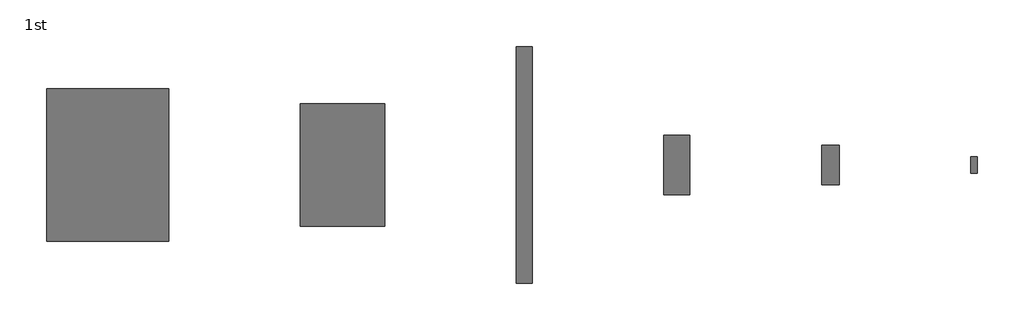
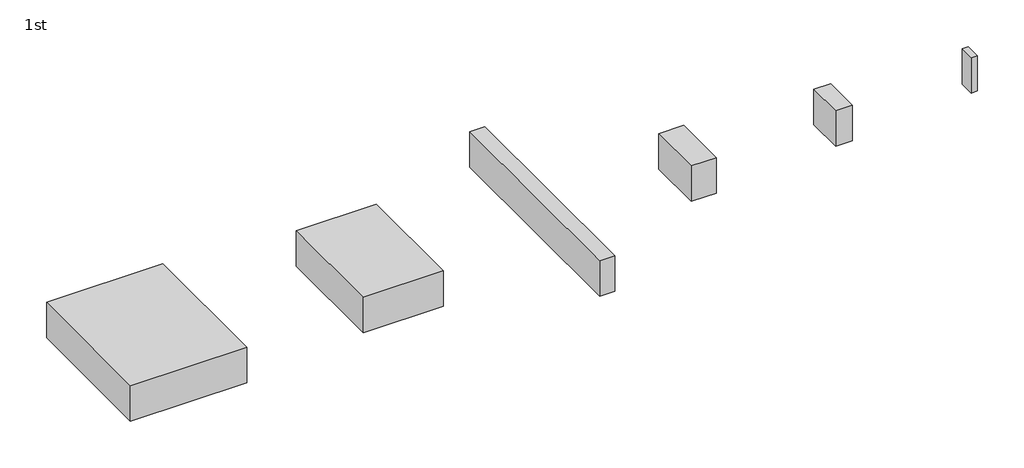
# One storey: 6 proxies.
"""IFC4 building model written with IfcOpenShell, lengths in millimetres."""

import ifcopenshell
import ifcopenshell.guid

model = None  # the IFC model being written
_history = None  # IfcOwnerHistory: only IFC2X3 demands one
_inside = {}  # id of a spatial element -> (the spatial element, [elements in it])
_under = {}  # id of a project, library or spatial element -> (it, [spatial elements below it])
_declared = {}  # id of a project -> (the project, [libraries it declares])
_typed = {}  # id of a type object -> (the type object, [elements of that type])
_made_of = {}  # id of a material, layer set ... -> (it, [elements and type objects made of it])


def new_model(schema):
    """Start an empty IFC model of exactly this schema.

    Asked for "IFC4X3", IfcOpenShell would pick the latest addendum, in which some entities
    have other attributes; the version numbers below select the first issue.
    IFC2X3 requires an IfcOwnerHistory on every rooted entity: one is made here for all.
    """
    global model, _history
    if schema == "IFC4X3":
        model = ifcopenshell.file(schema_version=(4, 3, 0, 0))
    else:
        model = ifcopenshell.file(schema=schema)
    _inside.clear()
    _under.clear()
    _declared.clear()
    _typed.clear()
    _made_of.clear()
    _history = None
    if model.schema == "IFC2X3":
        org = make("IfcOrganization", Name="unknown")
        user = make(
            "IfcPersonAndOrganization",
            ThePerson=make("IfcPerson", FamilyName="unknown"),
            TheOrganization=org,
        )
        app = make(
            "IfcApplication",
            ApplicationDeveloper=org,
            Version="unknown",
            ApplicationFullName="unknown",
            ApplicationIdentifier="unknown",
        )
        _history = make(
            "IfcOwnerHistory",
            OwningUser=user,
            OwningApplication=app,
            ChangeAction="ADDED",
            CreationDate=0,
        )
    return model


def make(cls, **values):
    """One entity of the class cls with the attributes given. An attribute that is None is left unset."""
    return model.create_entity(
        cls, **{name: value for name, value in values.items() if value is not None}
    )


def rooted(cls, **values):
    """An entity with a GlobalId (a new one), such as an element, a storey or a relation."""
    return make(cls, GlobalId=ifcopenshell.guid.new(), OwnerHistory=_history, **values)


def si_unit(unit_type, name, prefix=None):
    """IfcSIUnit, for example si_unit("LENGTHUNIT", "METRE", prefix="MILLI")."""
    return make("IfcSIUnit", UnitType=unit_type, Prefix=prefix, Name=name)


def assignment(units):
    """IfcUnitAssignment: the units of a project."""
    return None if units is None else make("IfcUnitAssignment", Units=units)


def point(xyz):
    """IfcCartesianPoint."""
    return None if xyz is None else make("IfcCartesianPoint", Coordinates=xyz)


def direction(xyz):
    """IfcDirection."""
    return None if xyz is None else make("IfcDirection", DirectionRatios=xyz)


def frame(location, z_axis=None, x_axis=None):
    """IfcAxis2Placement3D, a coordinate frame: its origin and axes. An axis left out is left unset."""
    return make(
        "IfcAxis2Placement3D",
        Location=point(location),
        Axis=direction(z_axis),
        RefDirection=direction(x_axis),
    )


def origin():
    """The frame at (0, 0, 0) with its axes left unset."""
    return frame((0.0, 0.0, 0.0))


def origin_with_axes():
    """The frame at (0, 0, 0) with the z axis (0, 0, 1) and the x axis (1, 0, 0) written out."""
    return frame((0.0, 0.0, 0.0), z_axis=(0.0, 0.0, 1.0), x_axis=(1.0, 0.0, 0.0))


def place(relative_to, where):
    """IfcLocalPlacement: puts the frame where relative to a parent placement (None: the world)."""
    return make(
        "IfcLocalPlacement", PlacementRelTo=relative_to, RelativePlacement=where
    )


def context(
    kind, dimensions, precision=None, world=None, true_north=None, identifier=None
):
    """IfcGeometricRepresentationContext, for example the 3D "Model" context."""
    return make(
        "IfcGeometricRepresentationContext",
        ContextIdentifier=identifier,
        ContextType=kind,
        CoordinateSpaceDimension=dimensions,
        Precision=precision,
        WorldCoordinateSystem=world,
        TrueNorth=true_north,
    )


def project(units=None, contexts=None):
    """IfcProject with its units and contexts."""
    return rooted(
        "IfcProject",
        Name="project",
        RepresentationContexts=contexts,
        UnitsInContext=assignment(units),
    )


def spatial(cls, under=None, at=None, **own):
    """A site, building, storey or space (cls), placed at a placement, below another one or the project."""
    s = rooted(cls, ObjectPlacement=at, **own)
    if under is not None:
        _under.setdefault(under.id(), (under, []))[1].append(s)
    return s


def polyline(points):
    """IfcPolyline through the points."""
    return make("IfcPolyline", Points=[point(p) for p in points])


def outline(outer, holes=None, kind="AREA"):
    """IfcArbitraryClosedProfileDef: a profile drawn as a closed curve; with holes, ...WithVoids."""
    if holes is None:
        return make("IfcArbitraryClosedProfileDef", ProfileType=kind, OuterCurve=outer)
    return make(
        "IfcArbitraryProfileDefWithVoids",
        ProfileType=kind,
        OuterCurve=outer,
        InnerCurves=holes,
    )


def extrude(swept, where, along, depth):
    """IfcExtrudedAreaSolid: the profile swept, set in the frame where, extruded along a direction by depth."""
    return make(
        "IfcExtrudedAreaSolid",
        SweptArea=swept,
        Position=where,
        ExtrudedDirection=direction(along),
        Depth=depth,
    )


def shape(context_of_items, identifier, shape_type, items):
    """IfcShapeRepresentation: the items that make up one representation, for example the "Body"."""
    return make(
        "IfcShapeRepresentation",
        ContextOfItems=context_of_items,
        RepresentationIdentifier=identifier,
        RepresentationType=shape_type,
        Items=items,
    )


def source(mapping_origin, context_of_items, identifier, shape_type, items):
    """IfcRepresentationMap: a shape defined once, which mapped items show again and again."""
    return make(
        "IfcRepresentationMap",
        MappingOrigin=mapping_origin,
        MappedRepresentation=shape(context_of_items, identifier, shape_type, items),
    )


def transform(
    local_origin,
    x_axis=None,
    y_axis=None,
    z_axis=None,
    scale=None,
    scale2=None,
    scale3=None,
    uniform=True,
):
    """IfcCartesianTransformationOperator3D, or its non-uniform kind. x_axis, y_axis, z_axis: its Axis1, 2, 3."""
    if uniform:
        return make(
            "IfcCartesianTransformationOperator3D",
            Axis1=direction(x_axis),
            Axis2=direction(y_axis),
            LocalOrigin=point(local_origin),
            Scale=scale,
            Axis3=direction(z_axis),
        )
    return make(
        "IfcCartesianTransformationOperator3DnonUniform",
        Axis1=direction(x_axis),
        Axis2=direction(y_axis),
        LocalOrigin=point(local_origin),
        Scale=scale,
        Axis3=direction(z_axis),
        Scale2=scale2,
        Scale3=scale3,
    )


def mapped(mapping_source, mapping_target):
    """IfcMappedItem: shows the shape of a source again, moved by a transform."""
    return make(
        "IfcMappedItem", MappingSource=mapping_source, MappingTarget=mapping_target
    )


def made_of(thing, what):
    """Note that an element or type object is made of a material, layer set ...; save() writes the relation."""
    if what is not None:
        _made_of.setdefault(what.id(), (what, []))[1].append(thing)
    return thing


def element(
    cls,
    number,
    at=None,
    inside=None,
    cuts=None,
    type_object=None,
    material=None,
    context=None,
    identifier="Body",
    shape_type=None,
    held_by="IfcProductDefinitionShape",
    body=None,
    shapes=None,
    **own,
):
    """One element of the class cls, such as IfcWall. Its Tag is "e" and its number.

    at: its placement. inside: the storey or other place that contains it. cuts: it is an
    opening in that element (IfcRelVoidsElement). A single representation is given by context,
    identifier, shape_type and body (its items); several are given by shapes. held_by: the class
    of the entity that holds the representations. save() writes the other relations.
    """
    e = rooted(cls, Tag="e%d" % number, ObjectPlacement=at, **own)
    if body is not None:
        shapes = [shape(context, identifier, shape_type, body)]
    if shapes is not None:
        e.Representation = make(held_by, Representations=shapes)
    if inside is not None:
        _inside.setdefault(inside.id(), (inside, []))[1].append(e)
    if cuts is not None:
        rooted(
            "IfcRelVoidsElement", RelatingBuildingElement=cuts, RelatedOpeningElement=e
        )
    if type_object is not None:
        _typed.setdefault(type_object.id(), (type_object, []))[1].append(e)
    return made_of(e, material)


def aggregate(whole, parts):
    """IfcRelAggregates: a whole, such as a stair, and the parts it consists of."""
    return rooted("IfcRelAggregates", RelatingObject=whole, RelatedObjects=parts)


def save(model, path):
    """Write the relations noted so far, then the file.

    IfcRelAggregates (storeys below a building ...), IfcRelContainedInSpatialStructure (elements
    in a storey), IfcRelDefinesByType, IfcRelAssociatesMaterial and IfcRelDeclares: one each for
    every whole, place, type object, material and project.
    """
    for whole, parts in _under.values():
        aggregate(whole, parts)
    for where, things in _inside.values():
        rooted(
            "IfcRelContainedInSpatialStructure",
            RelatedElements=things,
            RelatingStructure=where,
        )
    for kind, things in _typed.values():
        rooted("IfcRelDefinesByType", RelatedObjects=things, RelatingType=kind)
    for what, things in _made_of.values():
        rooted("IfcRelAssociatesMaterial", RelatedObjects=things, RelatingMaterial=what)
    for by, libraries in _declared.values():
        rooted("IfcRelDeclares", RelatingContext=by, RelatedDefinitions=libraries)
    model.write(path)


def generic_models_29bcd6f9(model_context):
    return source(origin(), model_context, "Body", "SweptSolid", [
        extrude(outline(polyline([(2000.0, 4500.0), (2000.0, -4500.0), (-2000.0, -4500.0), (-2000.0, 4500.0), (2000.0, 4500.0)])), origin_with_axes(), (0.0, 0.0, 1.0), 6000.0),
    ])


def generic_models_d82b1902(model_context):
    return source(origin(), model_context, "Body", "SweptSolid", [
        extrude(outline(polyline([(9300.0, 11600.0), (9300.0, -11600.0), (-9300.0, -11600.0), (-9300.0, 11600.0), (9300.0, 11600.0)])), origin_with_axes(), (0.0, 0.0, 1.0), 6000.0),
    ])


def generic_models_21711933(model_context):
    return source(origin(), model_context, "Body", "SweptSolid", [
        extrude(outline(polyline([(6400.0, 9300.0), (6400.0, -9300.0), (-6400.0, -9300.0), (-6400.0, 9300.0), (6400.0, 9300.0)])), origin_with_axes(), (0.0, 0.0, 1.0), 6000.0),
    ])


def generic_models_03d31222(model_context):
    return source(origin(), model_context, "Body", "SweptSolid", [
        extrude(outline(polyline([(1200.0, 18000.0), (1200.0, -18000.0), (-1200.0, -18000.0), (-1200.0, 18000.0), (1200.0, 18000.0)])), origin_with_axes(), (0.0, 0.0, 1.0), 6000.0),
    ])


def generic_models_5634f436(model_context):
    return source(origin(), model_context, "Body", "SweptSolid", [
        extrude(outline(polyline([(1350.0, 3000.0), (1350.0, -3000.0), (-1350.0, -3000.0), (-1350.0, 3000.0), (1350.0, 3000.0)])), origin_with_axes(), (0.0, 0.0, 1.0), 6000.0),
    ])


def generic_models_71e2440f(model_context):
    return source(origin(), model_context, "Body", "SweptSolid", [
        extrude(outline(polyline([(500.0, 1250.0), (500.0, -1250.0), (-500.0, -1250.0), (-500.0, 1250.0), (500.0, 1250.0)])), origin_with_axes(), (0.0, 0.0, 1.0), 6000.0),
    ])


model = new_model("IFC4")

# Units and contexts
model_context = context("Model", 3, world=origin())
ifc_project = project(units=[si_unit("LENGTHUNIT", "METRE", prefix="MILLI")], contexts=[model_context])

# Site, building, storey
site = spatial("IfcSite", under=ifc_project)
building = spatial("IfcBuilding", under=site)
storey = spatial("IfcBuildingStorey", under=building, Name="1st", Elevation=7000.0)

# Proxies
placement = place(None, origin())
generic_models_shape = generic_models_29bcd6f9(model_context)
element("IfcBuildingElementProxy", 1, Name="Space Planning Box_hec : Space Planning Box_hec", ObjectType="Space Planning Box_hec : Space Planning Box_hec", at=placement, inside=storey, context=model_context, shape_type="MappedRepresentation", body=[
    mapped(generic_models_shape, transform((95800.0, 114000.0, 7000.0), x_axis=(1.0, 0.0, 0.0), y_axis=(0.0, 1.0, 0.0), z_axis=(0.0, 0.0, 1.0))),
])
generic_models_2_shape = generic_models_d82b1902(model_context)
element("IfcBuildingElementProxy", 2, Name="Space Planning Box_hec : Space Planning Box_hec", ObjectType="Space Planning Box_hec : Space Planning Box_hec", at=placement, inside=storey, context=model_context, shape_type="MappedRepresentation", body=[
    mapped(generic_models_2_shape, transform((9300.0, 114000.0, 7000.0), x_axis=(1.0, 0.0, 0.0), y_axis=(0.0, 1.0, 0.0), z_axis=(0.0, 0.0, 1.0))),
])
generic_models_3_shape = generic_models_21711933(model_context)
element("IfcBuildingElementProxy", 3, Name="Space Planning Box_hec : Space Planning Box_hec", ObjectType="Space Planning Box_hec : Space Planning Box_hec", at=placement, inside=storey, context=model_context, shape_type="MappedRepresentation", body=[
    mapped(generic_models_3_shape, transform((45000.0, 114000.0, 7000.0), x_axis=(1.0, 0.0, 0.0), y_axis=(0.0, 1.0, 0.0), z_axis=(0.0, 0.0, 1.0))),
])
generic_models_4_shape = generic_models_03d31222(model_context)
element("IfcBuildingElementProxy", 4, Name="Space Planning Box_hec : Space Planning Box_hec", ObjectType="Space Planning Box_hec : Space Planning Box_hec", at=placement, inside=storey, context=model_context, shape_type="MappedRepresentation", body=[
    mapped(generic_models_4_shape, transform((72600.0, 114000.0, 7000.0), x_axis=(1.0, 0.0, 0.0), y_axis=(0.0, 1.0, 0.0), z_axis=(0.0, 0.0, 1.0))),
])
generic_models_5_shape = generic_models_5634f436(model_context)
element("IfcBuildingElementProxy", 5, Name="Space Planning Box_hec : Space Planning Box_hec", ObjectType="Space Planning Box_hec : Space Planning Box_hec", at=placement, inside=storey, context=model_context, shape_type="MappedRepresentation", body=[
    mapped(generic_models_5_shape, transform((119150.0, 114000.0, 7000.0), x_axis=(1.0, 0.0, 0.0), y_axis=(0.0, 1.0, 0.0), z_axis=(0.0, 0.0, 1.0))),
])
generic_models_6_shape = generic_models_71e2440f(model_context)
element("IfcBuildingElementProxy", 6, Name="Space Planning Box_hec : Space Planning Box_hec", ObjectType="Space Planning Box_hec : Space Planning Box_hec", at=placement, inside=storey, context=model_context, shape_type="MappedRepresentation", body=[
    mapped(generic_models_6_shape, transform((141000.0, 114000.0, 7000.0), x_axis=(1.0, 0.0, 0.0), y_axis=(0.0, 1.0, 0.0), z_axis=(0.0, 0.0, 1.0))),
])

save(model, "model.ifc")

# Revit data of these elements
# Project information
#   Project Issue Date = "Issue Date"
#   Project Status = "Project Status"
#   Client Name = "Owner"
#   Project Address = "Enter address here"
#   Project Name = "Project Name"
#   Project Number = "Project Number"
# Type "Space Planning Box_hec : Space Planning Box_hec"
#   Type Comments = "..."
#   Room Name [instance default] = "?"
#   Interior Finish [instance default] = ""
#   Exterior Finish [instance default] = ""
#   Department [instance default] = ""
#   Assembly Code = "..."
#   Width [instance default] = 1524 mm
#   Program Area [instance default] = 0 m²
#   Length [instance default] = 1524 mm
#   Height [instance default] = 1524 mm
#   Area [instance default] = 2.32258 m²
#   Fill Color [instance default] = Cyan
#   Default Elevation = 0
# Element 1 (IfcBuildingElementProxy, "Space Planning Box_hec : Space Planning Box_hec")
#   Room Name = "Stairway"
#   Interior Finish = "IF2"
#   Exterior Finish = "EF1"
#   Department = "AR"
#   Width = 4000 mm
#   Program Area = 36 m²
#   Length = 9000 mm
#   Height = 6000 mm
#   Area = 36 m²
#   Fill Color = Lavender
#   Phase Created = New Construction
#   Materials on its faces: "Lavender"
# Element 2 (IfcBuildingElementProxy, "Space Planning Box_hec : Space Planning Box_hec")
#   Room Name = "Electronic Room"
#   Interior Finish = "IF1"
#   Exterior Finish = "EF1"
#   Department = "CI"
#   Width = 18600 mm
#   Program Area = 431.52 m²
#   Length = 23200 mm
#   Height = 6000 mm
#   Area = 431.52 m²
#   Fill Color = Lime
#   Phase Created = New Construction
#   Materials on its faces: "Lime"
# Element 3 (IfcBuildingElementProxy, "Space Planning Box_hec : Space Planning Box_hec")
#   Room Name = "Electrical Room"
#   Interior Finish = "IF1"
#   Exterior Finish = "EF1"
#   Department = "EL"
#   Width = 12800 mm
#   Program Area = 238.08 m²
#   Length = 18600 mm
#   Height = 6000 mm
#   Area = 238.08 m²
#   Fill Color = Blue
#   Phase Created = New Construction
#   Materials on its faces: "Blue"
# Element 4 (IfcBuildingElementProxy, "Space Planning Box_hec : Space Planning Box_hec")
#   Room Name = "Corridor"
#   Interior Finish = "IF2-1"
#   Exterior Finish = "EF1"
#   Department = "AR"
#   Width = 2400 mm
#   Program Area = 86.4 m²
#   Length = 36000 mm
#   Height = 6000 mm
#   Area = 86.4 m²
#   Fill Color = Lavender
#   Phase Created = New Construction
#   Materials on its faces: "Lavender"
# Element 5 (IfcBuildingElementProxy, "Space Planning Box_hec : Space Planning Box_hec")
#   Room Name = "Duct Shaft"
#   Interior Finish = "NA"
#   Exterior Finish = "EF1"
#   Department = "HV"
#   Width = 2700 mm
#   Program Area = 16.2 m²
#   Length = 6000 mm
#   Height = 6000 mm
#   Area = 16.2 m²
#   Fill Color = Pink
#   Phase Created = New Construction
#   Materials on its faces: "Pink"
# Element 6 (IfcBuildingElementProxy, "Space Planning Box_hec : Space Planning Box_hec")
#   Room Name = "Pipe Shaft"
#   Interior Finish = "NA"
#   Exterior Finish = "EF1"
#   Department = "HV"
#   Width = 1000 mm
#   Program Area = 2.5 m²
#   Length = 2500 mm
#   Height = 6000 mm
#   Area = 2.5 m²
#   Fill Color = Pink
#   Phase Created = New Construction
#   Materials on its faces: "Pink"
# Materials
#   "Cyan": class "Generic", colour RGB 0 255 255, transparency 0.2, Cost = 0
#   "Lavender": class "Generic", colour RGB 186 85 211, transparency 0.2, Cost = 0
#   "Lime": class "Generic", colour RGB 0 255 0, transparency 0.2, Cost = 0
#   "Blue": class "Generic", colour RGB 0 0 255, transparency 0.2, Cost = 0
#   "Pink": class "Generic", colour RGB 255 105 180, transparency 0.2, Cost = 0
